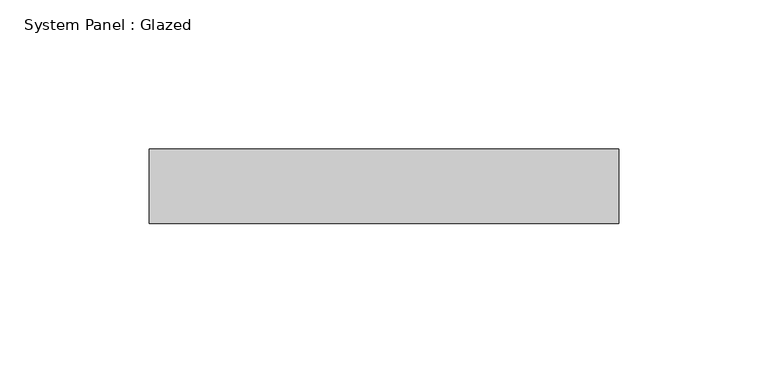
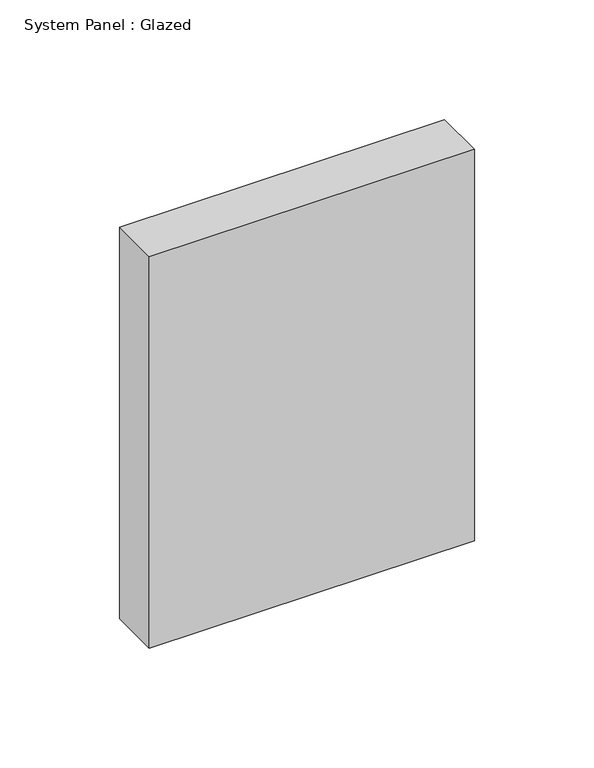
"""IFC4 building model written with IfcOpenShell, lengths in millimetres: plate geometry, System Panel : Glazed."""

from ifc_helpers import new_model, si_unit, origin, origin_with_axes, place, context, project, spatial, polyline, outline, extrude, source, transform, mapped, element, save


def system_panel_glazed_165eaad2(model_context):
    return source(origin(), model_context, "Body", "SweptSolid", [
        extrude(outline(polyline([(78.5977399, 24.5), (-78.5977399, 24.5), (-78.5977399, 49.5), (78.5977399, 49.5), (78.5977399, 24.5)])), origin_with_axes(), (0.0, 0.0, 1.0), 200.0),
    ])


if __name__ == "__main__":
    model = new_model("IFC4")
    model_context = context("Model", 3, world=origin())
    ifc_project = project(units=[si_unit("LENGTHUNIT", "METRE", prefix="MILLI")], contexts=[model_context])
    site = spatial("IfcSite", under=ifc_project)
    building = spatial("IfcBuilding", under=site)
    placement = place(None, origin())
    system_panel_glazed_shape = system_panel_glazed_165eaad2(model_context)
    element("IfcPlate", 1, ObjectType="System Panel : Glazed", at=placement, inside=building, context=model_context, shape_type="MappedRepresentation", body=[
        mapped(system_panel_glazed_shape, transform((0.0, 0.0, 0.0), x_axis=(1.0, 0.0, 0.0), y_axis=(0.0, 1.0, 0.0), z_axis=(0.0, 0.0, 1.0))),
    ])
    save(model, "model.ifc")

# Revit data of these elements
# Element 1 (IfcPlate, "System Panel : Glazed")
#   Materials on its faces: "Glass"
# Materials
#   "Glass": class "Glass", colour RGB 218 227 224, transparency 0.85, Description = "Soda Lime Glass", Cost = 0
